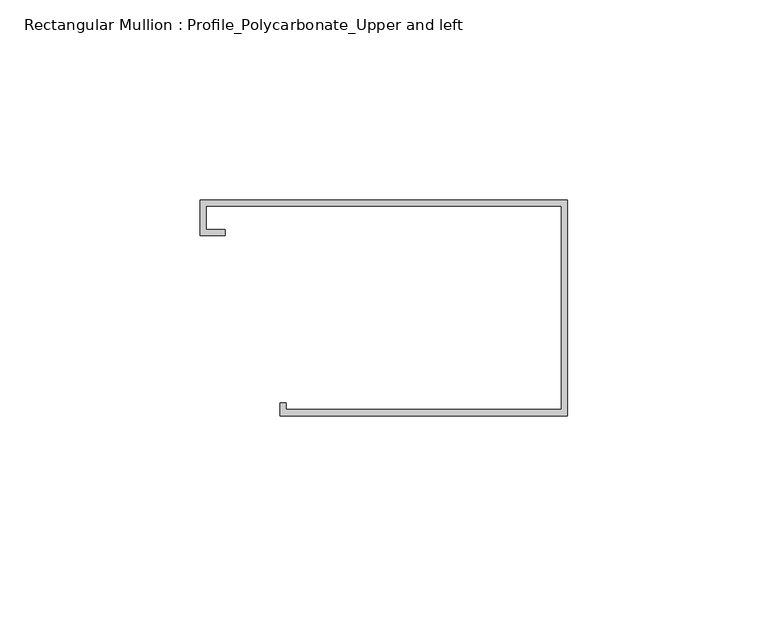
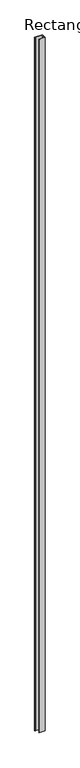
"""IFC4 building model written with IfcOpenShell, lengths in millimetres: member geometry, Rectangular Mullion : Profile_Polycarbonate_Upper and left."""

from ifc_helpers import new_model, si_unit, frame, origin, place, context, project, spatial, polyline, outline, extrude, source, transform, mapped, element, save


def rectangular_mullion_profile_polycarbonate_upper_and_left_ffa349e6(model_context):
    return source(origin(), model_context, "Body", "SweptSolid", [
        extrude(outline(polyline([(0.0, 28.984575), (0.0, -25.015825), (-71.9836, -25.015825), (-71.9836, -21.840825), (-70.3961, -21.840825), (-70.3961, -23.428325), (-1.5875, -23.428325), (-1.5875, 27.397075), (-90.4113, 27.397075), (-90.4113, 21.580475), (-85.6488, 21.580475), (-85.6488, 19.992975), (-91.9988, 19.992975), (-91.9988, 28.984575), (0.0, 28.984575)])), frame((0.0, 0.0, -8839.2), z_axis=(0.0, 0.0, 1.0), x_axis=(1.0, 0.0, 0.0)), (0.0, 0.0, 1.0), 8839.2),
    ])


if __name__ == "__main__":
    model = new_model("IFC4")
    model_context = context("Model", 3, world=origin())
    ifc_project = project(units=[si_unit("LENGTHUNIT", "METRE", prefix="MILLI")], contexts=[model_context])
    site = spatial("IfcSite", under=ifc_project)
    building = spatial("IfcBuilding", under=site)
    placement = place(None, origin())
    rectangular_mullion_profile_polycarbonate_upper_and_left_shape = rectangular_mullion_profile_polycarbonate_upper_and_left_ffa349e6(model_context)
    element("IfcMember", 1, ObjectType="Rectangular Mullion : Profile_Polycarbonate_Upper and left", at=placement, inside=building, context=model_context, shape_type="MappedRepresentation", body=[
        mapped(rectangular_mullion_profile_polycarbonate_upper_and_left_shape, transform((0.0, 0.0, 0.0), x_axis=(1.0, 0.0, 0.0), y_axis=(0.0, 1.0, 0.0), z_axis=(0.0, 0.0, 1.0))),
    ])
    save(model, "model.ifc")

# Revit data of these elements
# Type "Rectangular Mullion : Profile_Polycarbonate_Upper and left"
#   built-in parameter 1007322 = 0.177167 (stored number, unit not read)
#   built-in parameter 1007321 = 0.00520833 (stored number, unit not read)
#   built-in parameter 1007320 = 0 (stored number, unit not read)
